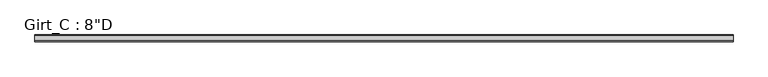
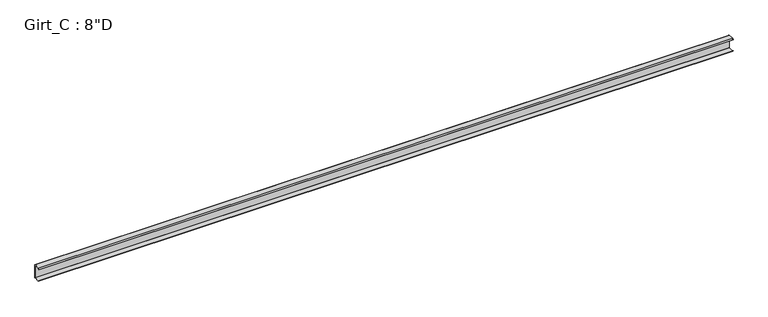
"""IFC4 building model written with IfcOpenShell, lengths in millimetres: beam geometry."""

from ifc_helpers import new_model, si_unit, point, frame, frame_2d, origin, place, context, project, spatial, polyline, circle_curve, trimmed, segment, composite_curve, outline, extrude, source, transform, mapped, element, save


def beam_0767d56c(model_context):
    return source(origin(), model_context, "Body", "SweptSolid", [
        extrude(outline(composite_curve([segment(polyline([(-87.5109375, 101.6), (-3.3734375, 101.6)]), True, "CONTINUOUS"), segment(trimmed(circle_curve(frame_2d((-3.3734375, 96.8375)), 4.7625), [point((-3.3734375, 101.6))], [point((1.3890625, 96.8375))], False, "CARTESIAN"), True, "CONTINUOUS"), segment(polyline([(1.3890625, 96.8375), (1.3890625, -96.8375)]), True, "CONTINUOUS"), segment(trimmed(circle_curve(frame_2d((-3.3734375, -96.8375)), 4.7625), [point((1.3890625, -96.8375))], [point((-3.3734375, -101.6))], False, "CARTESIAN"), True, "CONTINUOUS"), segment(polyline([(-3.3734375, -101.6), (-87.5109375, -101.6), (-99.7792647, -86.979177), (-97.6510975, -85.1934327), (-86.2154765, -98.821875), (-3.2694106, -98.821875)]), True, "CONTINUOUS"), segment(trimmed(circle_curve(frame_2d((-3.3748024, -96.8389339)), 1.9857399), [point((-3.2694106, -98.821875))], [point((-1.3890625, -96.8389339))], True, "CARTESIAN"), True, "CONTINUOUS"), segment(polyline([(-1.3890625, -96.8389339), (-1.3890625, 96.8381931)]), True, "CONTINUOUS"), segment(trimmed(circle_curve(frame_2d((-3.3741066, 96.8381931)), 1.9850441), [point((-1.3890625, 96.8381931))], [point((-3.3005807, 98.821875))], True, "CARTESIAN"), True, "CONTINUOUS"), segment(polyline([(-3.3005807, 98.821875), (-86.2154765, 98.821875), (-97.6278742, 85.221109), (-99.7560415, 87.0068534), (-87.5109375, 101.6)]), True, "CONTINUOUS")], self_intersect=False)), frame((-5133.2765, 0.0, 0.0), z_axis=(1.0, 0.0, 0.0), x_axis=(0.0, 1.0, 0.0)), (0.0, 0.0, 1.0), 10279.253),
    ])


if __name__ == "__main__":
    model = new_model("IFC4")
    model_context = context("Model", 3, world=origin())
    ifc_project = project(units=[si_unit("LENGTHUNIT", "METRE", prefix="MILLI")], contexts=[model_context])
    site = spatial("IfcSite", under=ifc_project)
    building = spatial("IfcBuilding", under=site)
    placement = place(None, origin())
    beam_shape = beam_0767d56c(model_context)
    element("IfcBeam", 1, ObjectType="Girt_C : 8\"D", at=placement, inside=building, context=model_context, shape_type="MappedRepresentation", body=[
        mapped(beam_shape, transform((0.0, 0.0, 0.0), x_axis=(1.0, 0.0, 0.0), y_axis=(0.0, 1.0, 0.0), z_axis=(0.0, 0.0, 1.0))),
    ])
    save(model, "model.ifc")

# Revit data of these elements
# Type "Girt_C : 8\"D"
#   half leg = 0' - 1 3/4"
#   Web_Thickness = 0' - 0 7/64"
#   Length [instance default] = 10' - 0"
#   Leg_1 = 0' - 3 1/2"
#   Height = 0' - 8"
#   Structural Material [instance default] = none
# Element 1 (IfcBeam, "Girt_C : 8\"D")
#   Materials on its faces: "CEE' SECTION (8.0x3.5C - SEE STRUCT. DWGS)"
# Materials
#   "CEE' SECTION (8.0x3.5C - SEE STRUCT. DWGS)": class "Metal", colour RGB 137 146 153, transparency 0, Description = "Steel, mill finish", Cost = 0
